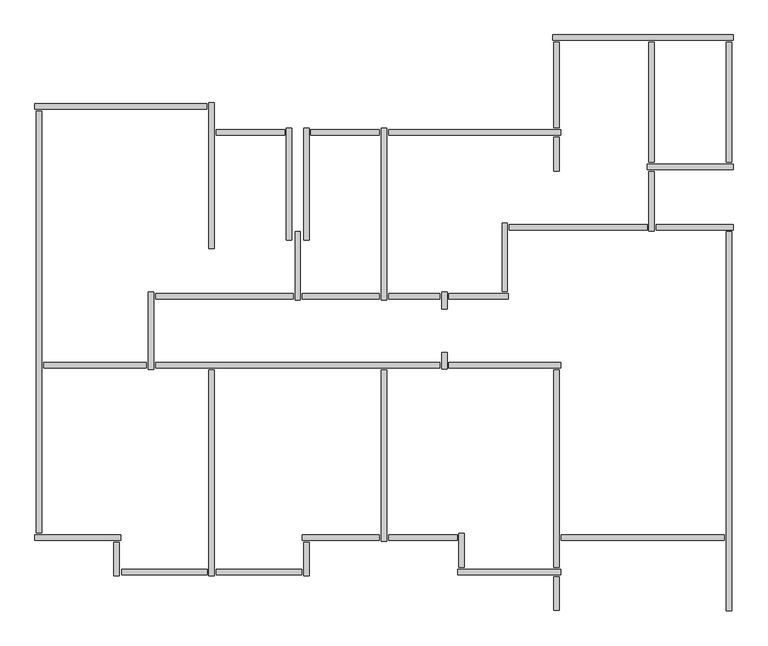
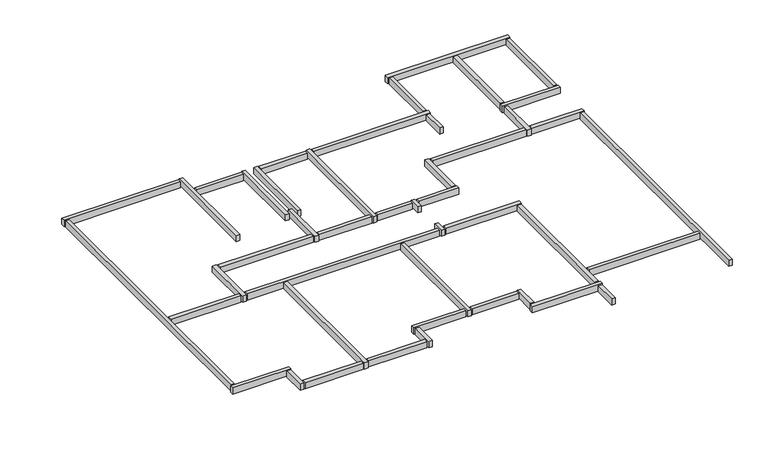
"""IFC4 building model written with IfcOpenShell, lengths in millimetres: beam geometry, Graute viga de respaldo2 : Graute viga de respaldo."""

import ifcopenshell
import ifcopenshell.guid

model = None  # the IFC model being written
_history = None  # IfcOwnerHistory: only IFC2X3 demands one
_inside = {}  # id of a spatial element -> (the spatial element, [elements in it])
_under = {}  # id of a project, library or spatial element -> (it, [spatial elements below it])
_declared = {}  # id of a project -> (the project, [libraries it declares])
_typed = {}  # id of a type object -> (the type object, [elements of that type])
_made_of = {}  # id of a material, layer set ... -> (it, [elements and type objects made of it])


def new_model(schema):
    """Start an empty IFC model of exactly this schema.

    Asked for "IFC4X3", IfcOpenShell would pick the latest addendum, in which some entities
    have other attributes; the version numbers below select the first issue.
    IFC2X3 requires an IfcOwnerHistory on every rooted entity: one is made here for all.
    """
    global model, _history
    if schema == "IFC4X3":
        model = ifcopenshell.file(schema_version=(4, 3, 0, 0))
    else:
        model = ifcopenshell.file(schema=schema)
    _inside.clear()
    _under.clear()
    _declared.clear()
    _typed.clear()
    _made_of.clear()
    _history = None
    if model.schema == "IFC2X3":
        org = make("IfcOrganization", Name="unknown")
        user = make(
            "IfcPersonAndOrganization",
            ThePerson=make("IfcPerson", FamilyName="unknown"),
            TheOrganization=org,
        )
        app = make(
            "IfcApplication",
            ApplicationDeveloper=org,
            Version="unknown",
            ApplicationFullName="unknown",
            ApplicationIdentifier="unknown",
        )
        _history = make(
            "IfcOwnerHistory",
            OwningUser=user,
            OwningApplication=app,
            ChangeAction="ADDED",
            CreationDate=0,
        )
    return model


def make(cls, **values):
    """One entity of the class cls with the attributes given. An attribute that is None is left unset."""
    return model.create_entity(
        cls, **{name: value for name, value in values.items() if value is not None}
    )


def rooted(cls, **values):
    """An entity with a GlobalId (a new one), such as an element, a storey or a relation."""
    return make(cls, GlobalId=ifcopenshell.guid.new(), OwnerHistory=_history, **values)


def si_unit(unit_type, name, prefix=None):
    """IfcSIUnit, for example si_unit("LENGTHUNIT", "METRE", prefix="MILLI")."""
    return make("IfcSIUnit", UnitType=unit_type, Prefix=prefix, Name=name)


def assignment(units):
    """IfcUnitAssignment: the units of a project."""
    return None if units is None else make("IfcUnitAssignment", Units=units)


def point(xyz):
    """IfcCartesianPoint."""
    return None if xyz is None else make("IfcCartesianPoint", Coordinates=xyz)


def direction(xyz):
    """IfcDirection."""
    return None if xyz is None else make("IfcDirection", DirectionRatios=xyz)


def frame(location, z_axis=None, x_axis=None):
    """IfcAxis2Placement3D, a coordinate frame: its origin and axes. An axis left out is left unset."""
    return make(
        "IfcAxis2Placement3D",
        Location=point(location),
        Axis=direction(z_axis),
        RefDirection=direction(x_axis),
    )


def origin():
    """The frame at (0, 0, 0) with its axes left unset."""
    return frame((0.0, 0.0, 0.0))


def place(relative_to, where):
    """IfcLocalPlacement: puts the frame where relative to a parent placement (None: the world)."""
    return make(
        "IfcLocalPlacement", PlacementRelTo=relative_to, RelativePlacement=where
    )


def context(
    kind, dimensions, precision=None, world=None, true_north=None, identifier=None
):
    """IfcGeometricRepresentationContext, for example the 3D "Model" context."""
    return make(
        "IfcGeometricRepresentationContext",
        ContextIdentifier=identifier,
        ContextType=kind,
        CoordinateSpaceDimension=dimensions,
        Precision=precision,
        WorldCoordinateSystem=world,
        TrueNorth=true_north,
    )


def project(units=None, contexts=None):
    """IfcProject with its units and contexts."""
    return rooted(
        "IfcProject",
        Name="project",
        RepresentationContexts=contexts,
        UnitsInContext=assignment(units),
    )


def spatial(cls, under=None, at=None, **own):
    """A site, building, storey or space (cls), placed at a placement, below another one or the project."""
    s = rooted(cls, ObjectPlacement=at, **own)
    if under is not None:
        _under.setdefault(under.id(), (under, []))[1].append(s)
    return s


def polyline(points):
    """IfcPolyline through the points."""
    return make("IfcPolyline", Points=[point(p) for p in points])


def outline(outer, holes=None, kind="AREA"):
    """IfcArbitraryClosedProfileDef: a profile drawn as a closed curve; with holes, ...WithVoids."""
    if holes is None:
        return make("IfcArbitraryClosedProfileDef", ProfileType=kind, OuterCurve=outer)
    return make(
        "IfcArbitraryProfileDefWithVoids",
        ProfileType=kind,
        OuterCurve=outer,
        InnerCurves=holes,
    )


def extrude(swept, where, along, depth):
    """IfcExtrudedAreaSolid: the profile swept, set in the frame where, extruded along a direction by depth."""
    return make(
        "IfcExtrudedAreaSolid",
        SweptArea=swept,
        Position=where,
        ExtrudedDirection=direction(along),
        Depth=depth,
    )


def shape(context_of_items, identifier, shape_type, items):
    """IfcShapeRepresentation: the items that make up one representation, for example the "Body"."""
    return make(
        "IfcShapeRepresentation",
        ContextOfItems=context_of_items,
        RepresentationIdentifier=identifier,
        RepresentationType=shape_type,
        Items=items,
    )


def source(mapping_origin, context_of_items, identifier, shape_type, items):
    """IfcRepresentationMap: a shape defined once, which mapped items show again and again."""
    return make(
        "IfcRepresentationMap",
        MappingOrigin=mapping_origin,
        MappedRepresentation=shape(context_of_items, identifier, shape_type, items),
    )


def transform(
    local_origin,
    x_axis=None,
    y_axis=None,
    z_axis=None,
    scale=None,
    scale2=None,
    scale3=None,
    uniform=True,
):
    """IfcCartesianTransformationOperator3D, or its non-uniform kind. x_axis, y_axis, z_axis: its Axis1, 2, 3."""
    if uniform:
        return make(
            "IfcCartesianTransformationOperator3D",
            Axis1=direction(x_axis),
            Axis2=direction(y_axis),
            LocalOrigin=point(local_origin),
            Scale=scale,
            Axis3=direction(z_axis),
        )
    return make(
        "IfcCartesianTransformationOperator3DnonUniform",
        Axis1=direction(x_axis),
        Axis2=direction(y_axis),
        LocalOrigin=point(local_origin),
        Scale=scale,
        Axis3=direction(z_axis),
        Scale2=scale2,
        Scale3=scale3,
    )


def mapped(mapping_source, mapping_target):
    """IfcMappedItem: shows the shape of a source again, moved by a transform."""
    return make(
        "IfcMappedItem", MappingSource=mapping_source, MappingTarget=mapping_target
    )


def made_of(thing, what):
    """Note that an element or type object is made of a material, layer set ...; save() writes the relation."""
    if what is not None:
        _made_of.setdefault(what.id(), (what, []))[1].append(thing)
    return thing


def element(
    cls,
    number,
    at=None,
    inside=None,
    cuts=None,
    type_object=None,
    material=None,
    context=None,
    identifier="Body",
    shape_type=None,
    held_by="IfcProductDefinitionShape",
    body=None,
    shapes=None,
    **own,
):
    """One element of the class cls, such as IfcWall. Its Tag is "e" and its number.

    at: its placement. inside: the storey or other place that contains it. cuts: it is an
    opening in that element (IfcRelVoidsElement). A single representation is given by context,
    identifier, shape_type and body (its items); several are given by shapes. held_by: the class
    of the entity that holds the representations. save() writes the other relations.
    """
    e = rooted(cls, Tag="e%d" % number, ObjectPlacement=at, **own)
    if body is not None:
        shapes = [shape(context, identifier, shape_type, body)]
    if shapes is not None:
        e.Representation = make(held_by, Representations=shapes)
    if inside is not None:
        _inside.setdefault(inside.id(), (inside, []))[1].append(e)
    if cuts is not None:
        rooted(
            "IfcRelVoidsElement", RelatingBuildingElement=cuts, RelatedOpeningElement=e
        )
    if type_object is not None:
        _typed.setdefault(type_object.id(), (type_object, []))[1].append(e)
    return made_of(e, material)


def aggregate(whole, parts):
    """IfcRelAggregates: a whole, such as a stair, and the parts it consists of."""
    return rooted("IfcRelAggregates", RelatingObject=whole, RelatedObjects=parts)


def save(model, path):
    """Write the relations noted so far, then the file.

    IfcRelAggregates (storeys below a building ...), IfcRelContainedInSpatialStructure (elements
    in a storey), IfcRelDefinesByType, IfcRelAssociatesMaterial and IfcRelDeclares: one each for
    every whole, place, type object, material and project.
    """
    for whole, parts in _under.values():
        aggregate(whole, parts)
    for where, things in _inside.values():
        rooted(
            "IfcRelContainedInSpatialStructure",
            RelatedElements=things,
            RelatingStructure=where,
        )
    for kind, things in _typed.values():
        rooted("IfcRelDefinesByType", RelatedObjects=things, RelatingType=kind)
    for what, things in _made_of.values():
        rooted("IfcRelAssociatesMaterial", RelatedObjects=things, RelatingMaterial=what)
    for by, libraries in _declared.values():
        rooted("IfcRelDeclares", RelatingContext=by, RelatedDefinitions=libraries)
    model.write(path)


def beam_834ff979(model_context):
    return source(origin(), model_context, "Body", "SweptSolid", [
        extrude(outline(polyline([(-75401.7587292, 57502.4278788), (-75401.7587292, 57408.4278788), (-76591.7587292, 57408.4278788), (-76591.7587292, 57502.4278788), (-75401.7587292, 57502.4278788)])), frame((0.0, 0.0, 2632.9999999), z_axis=(0.0, 0.0, 1.0), x_axis=(1.0, 0.0, 0.0)), (0.0, 0.0, 1.0), 167.0),
        extrude(outline(polyline([(-73751.7587292, 57502.4278788), (-73751.7587292, 57408.4278788), (-74941.7587292, 57408.4278788), (-74941.7587292, 57502.4278788), (-73751.7587292, 57502.4278788)])), frame((0.0, 0.0, 2632.9999999), z_axis=(0.0, 0.0, 1.0), x_axis=(1.0, 0.0, 0.0)), (0.0, 0.0, 1.0), 167.0),
        extrude(outline(polyline([(-77801.7587292, 53452.4278788), (-77801.7587292, 53358.4278788), (-79591.7587292, 53358.4278788), (-79591.7587292, 53452.4278788), (-77801.7587292, 53452.4278788)])), frame((0.0, 0.0, 2632.9999999), z_axis=(0.0, 0.0, 1.0), x_axis=(1.0, 0.0, 0.0)), (0.0, 0.0, 1.0), 167.0),
        extrude(outline(polyline([(-72401.7587292, 50452.4278788), (-72401.7587292, 50358.4278788), (-73591.7587292, 50358.4278788), (-73591.7587292, 50452.4278788), (-72401.7587292, 50452.4278788)])), frame((0.0, 0.0, 2632.9999999), z_axis=(0.0, 0.0, 1.0), x_axis=(1.0, 0.0, 0.0)), (0.0, 0.0, 1.0), 167.0),
        extrude(outline(polyline([(-72368.7587292, 50475.4278788), (-72274.7587292, 50475.4278788), (-72274.7587292, 49885.4278788), (-72368.7587292, 49885.4278788), (-72368.7587292, 50475.4278788)])), frame((0.0, 0.0, 2632.9999999), z_axis=(0.0, 0.0, 1.0), x_axis=(1.0, 0.0, 0.0)), (0.0, 0.0, 1.0), 167.0),
        extrude(outline(polyline([(-70601.7587292, 49852.4278788), (-70601.7587292, 49758.4278788), (-72391.7587292, 49758.4278788), (-72391.7587292, 49852.4278788), (-70601.7587292, 49852.4278788)])), frame((0.0, 0.0, 2632.9999999), z_axis=(0.0, 0.0, 1.0), x_axis=(1.0, 0.0, 0.0)), (0.0, 0.0, 1.0), 167.0),
        extrude(outline(polyline([(-72574.7587292, 53335.4278788), (-72668.7587292, 53335.4278788), (-72668.7587292, 53625.4278788), (-72574.7587292, 53625.4278788), (-72574.7587292, 53335.4278788)])), frame((0.0, 0.0, 2632.9999999), z_axis=(0.0, 0.0, 1.0), x_axis=(1.0, 0.0, 0.0)), (0.0, 0.0, 1.0), 167.0),
        extrude(outline(polyline([(-75251.7587292, 54652.4278788), (-75251.7587292, 54558.4278788), (-77641.7587292, 54558.4278788), (-77641.7587292, 54652.4278788), (-75251.7587292, 54652.4278788)])), frame((0.0, 0.0, 2632.9999999), z_axis=(0.0, 0.0, 1.0), x_axis=(1.0, 0.0, 0.0)), (0.0, 0.0, 1.0), 167.0),
        extrude(outline(polyline([(-73751.7587292, 54652.4278788), (-73751.7587292, 54558.4278788), (-75091.7587292, 54558.4278788), (-75091.7587292, 54652.4278788), (-73751.7587292, 54652.4278788)])), frame((0.0, 0.0, 2632.9999999), z_axis=(0.0, 0.0, 1.0), x_axis=(1.0, 0.0, 0.0)), (0.0, 0.0, 1.0), 167.0),
        extrude(outline(polyline([(-72701.7587292, 54652.4278788), (-72701.7587292, 54558.4278788), (-73591.7587292, 54558.4278788), (-73591.7587292, 54652.4278788), (-72701.7587292, 54652.4278788)])), frame((0.0, 0.0, 2632.9999999), z_axis=(0.0, 0.0, 1.0), x_axis=(1.0, 0.0, 0.0)), (0.0, 0.0, 1.0), 167.0),
        extrude(outline(polyline([(-72574.7587292, 54385.4278788), (-72668.7587292, 54385.4278788), (-72668.7587292, 54675.4278788), (-72574.7587292, 54675.4278788), (-72574.7587292, 54385.4278788)])), frame((0.0, 0.0, 2632.9999999), z_axis=(0.0, 0.0, 1.0), x_axis=(1.0, 0.0, 0.0)), (0.0, 0.0, 1.0), 167.0),
        extrude(outline(polyline([(-71511.7587292, 54652.4278788), (-71511.7587292, 54558.4278788), (-72541.7587292, 54558.4278788), (-72541.7587292, 54652.4278788), (-71511.7587292, 54652.4278788)])), frame((0.0, 0.0, 2632.9999999), z_axis=(0.0, 0.0, 1.0), x_axis=(1.0, 0.0, 0.0)), (0.0, 0.0, 1.0), 167.0),
        extrude(outline(polyline([(-71618.7587292, 55875.4278788), (-71524.7587292, 55875.4278788), (-71524.7587292, 54685.4278788), (-71618.7587292, 54685.4278788), (-71618.7587292, 55875.4278788)])), frame((0.0, 0.0, 2632.9999999), z_axis=(0.0, 0.0, 1.0), x_axis=(1.0, 0.0, 0.0)), (0.0, 0.0, 1.0), 167.0),
        extrude(outline(polyline([(-69091.7587292, 55852.4278788), (-69091.7587292, 55758.4278788), (-71491.7587292, 55758.4278788), (-71491.7587292, 55852.4278788), (-69091.7587292, 55852.4278788)])), frame((0.0, 0.0, 2632.9999999), z_axis=(0.0, 0.0, 1.0), x_axis=(1.0, 0.0, 0.0)), (0.0, 0.0, 1.0), 167.0),
        extrude(outline(polyline([(-73624.7587292, 54540.4278788), (-73718.7587292, 54540.4278788), (-73718.7587292, 57525.4278788), (-73624.7587292, 57525.4278788), (-73624.7587292, 54540.4278788)])), frame((0.0, 0.0, 2632.9999999), z_axis=(0.0, 0.0, 1.0), x_axis=(1.0, 0.0, 0.0)), (0.0, 0.0, 1.0), 167.0),
        extrude(outline(polyline([(-70601.7587292, 57502.4278788), (-70601.7587292, 57408.4278788), (-73591.7587292, 57408.4278788), (-73591.7587292, 57502.4278788), (-70601.7587292, 57502.4278788)])), frame((0.0, 0.0, 2632.9999999), z_axis=(0.0, 0.0, 1.0), x_axis=(1.0, 0.0, 0.0)), (0.0, 0.0, 1.0), 167.0),
        extrude(outline(polyline([(-70624.7587292, 56785.4278788), (-70718.7587292, 56785.4278788), (-70718.7587292, 57375.4278788), (-70624.7587292, 57375.4278788), (-70624.7587292, 56785.4278788)])), frame((0.0, 0.0, 2632.9999999), z_axis=(0.0, 0.0, 1.0), x_axis=(1.0, 0.0, 0.0)), (0.0, 0.0, 1.0), 167.0),
        extrude(outline(polyline([(-70718.7587292, 59025.4278788), (-70624.7587292, 59025.4278788), (-70624.7587292, 57535.4278788), (-70718.7587292, 57535.4278788), (-70718.7587292, 59025.4278788)])), frame((0.0, 0.0, 2632.9999999), z_axis=(0.0, 0.0, 1.0), x_axis=(1.0, 0.0, 0.0)), (0.0, 0.0, 1.0), 167.0),
        extrude(outline(polyline([(-67718.7587292, 59025.4278788), (-67624.7587292, 59025.4278788), (-67624.7587292, 56935.4278788), (-67718.7587292, 56935.4278788), (-67718.7587292, 59025.4278788)])), frame((0.0, 0.0, 2632.9999999), z_axis=(0.0, 0.0, 1.0), x_axis=(1.0, 0.0, 0.0)), (0.0, 0.0, 1.0), 167.0),
        extrude(outline(polyline([(-69068.7587292, 59025.4278788), (-68974.7587292, 59025.4278788), (-68974.7587292, 56935.4278788), (-69068.7587292, 56935.4278788), (-69068.7587292, 59025.4278788)])), frame((0.0, 0.0, 2632.9999999), z_axis=(0.0, 0.0, 1.0), x_axis=(1.0, 0.0, 0.0)), (0.0, 0.0, 1.0), 167.0),
        extrude(outline(polyline([(-68974.7587292, 55735.4278788), (-69068.7587292, 55735.4278788), (-69068.7587292, 56775.4278788), (-68974.7587292, 56775.4278788), (-68974.7587292, 55735.4278788)])), frame((0.0, 0.0, 2632.9999999), z_axis=(0.0, 0.0, 1.0), x_axis=(1.0, 0.0, 0.0)), (0.0, 0.0, 1.0), 167.0),
        extrude(outline(polyline([(-67751.7587292, 50452.4278788), (-67751.7587292, 50358.4278788), (-70591.7587292, 50358.4278788), (-70591.7587292, 50452.4278788), (-67751.7587292, 50452.4278788)])), frame((0.0, 0.0, 2632.9999999), z_axis=(0.0, 0.0, 1.0), x_axis=(1.0, 0.0, 0.0)), (0.0, 0.0, 1.0), 167.0),
        extrude(outline(polyline([(-70718.7587292, 53325.4278788), (-70624.7587292, 53325.4278788), (-70624.7587292, 49885.4278788), (-70718.7587292, 49885.4278788), (-70718.7587292, 53325.4278788)])), frame((0.0, 0.0, 2632.9999999), z_axis=(0.0, 0.0, 1.0), x_axis=(1.0, 0.0, 0.0)), (0.0, 0.0, 1.0), 167.0),
        extrude(outline(polyline([(-70601.7587292, 53452.4278788), (-70601.7587292, 53358.4278788), (-72541.7587292, 53358.4278788), (-72541.7587292, 53452.4278788), (-70601.7587292, 53452.4278788)])), frame((0.0, 0.0, 2632.9999999), z_axis=(0.0, 0.0, 1.0), x_axis=(1.0, 0.0, 0.0)), (0.0, 0.0, 1.0), 167.0),
        extrude(outline(polyline([(-72701.7587292, 53452.4278788), (-72701.7587292, 53358.4278788), (-77641.7587292, 53358.4278788), (-77641.7587292, 53452.4278788), (-72701.7587292, 53452.4278788)])), frame((0.0, 0.0, 2632.9999999), z_axis=(0.0, 0.0, 1.0), x_axis=(1.0, 0.0, 0.0)), (0.0, 0.0, 1.0), 167.0),
        extrude(outline(polyline([(-73624.7587292, 50335.4278788), (-73718.7587292, 50335.4278788), (-73718.7587292, 53325.4278788), (-73624.7587292, 53325.4278788), (-73624.7587292, 50335.4278788)])), frame((0.0, 0.0, 2632.9999999), z_axis=(0.0, 0.0, 1.0), x_axis=(1.0, 0.0, 0.0)), (0.0, 0.0, 1.0), 167.0),
        extrude(outline(polyline([(-75091.7587292, 50358.4278788), (-75091.7587292, 50452.4278788), (-73751.7587292, 50452.4278788), (-73751.7587292, 50358.4278788), (-75091.7587292, 50358.4278788)])), frame((0.0, 0.0, 2632.9999999), z_axis=(0.0, 0.0, 1.0), x_axis=(1.0, 0.0, 0.0)), (0.0, 0.0, 1.0), 167.0),
        extrude(outline(polyline([(-74974.7587292, 49735.4278788), (-75068.7587292, 49735.4278788), (-75068.7587292, 50325.4278788), (-74974.7587292, 50325.4278788), (-74974.7587292, 49735.4278788)])), frame((0.0, 0.0, 2632.9999999), z_axis=(0.0, 0.0, 1.0), x_axis=(1.0, 0.0, 0.0)), (0.0, 0.0, 1.0), 167.0),
        extrude(outline(polyline([(-75101.7587292, 49852.4278788), (-75101.7587292, 49758.4278788), (-76591.7587292, 49758.4278788), (-76591.7587292, 49852.4278788), (-75101.7587292, 49852.4278788)])), frame((0.0, 0.0, 2632.9999999), z_axis=(0.0, 0.0, 1.0), x_axis=(1.0, 0.0, 0.0)), (0.0, 0.0, 1.0), 167.0),
        extrude(outline(polyline([(-78230.736554, 49758.4278788), (-78230.736554, 49853.4278788), (-76741.7587292, 49853.4278788), (-76741.7587292, 49758.4278788), (-78230.736554, 49758.4278788)])), frame((0.0, 0.0, 2617.1856208), z_axis=(0.0, 0.0, 1.0), x_axis=(1.0, 0.0, 0.0)), (0.0, 0.0, 1.0), 165.0),
        extrude(outline(polyline([(-79718.7587292, 57825.4278788), (-79624.7587292, 57825.4278788), (-79624.7587292, 50485.4278788), (-79718.7587292, 50485.4278788), (-79718.7587292, 57825.4278788)])), frame((0.0, 0.0, 2632.9999999), z_axis=(0.0, 0.0, 1.0), x_axis=(1.0, 0.0, 0.0)), (0.0, 0.0, 1.0), 167.0),
        extrude(outline(polyline([(-77768.7587292, 54675.4278788), (-77674.7587292, 54675.4278788), (-77674.7587292, 53330.0746661), (-77768.7587292, 53330.0746661), (-77768.7587292, 54675.4278788)])), frame((0.0, 0.0, 2632.9999999), z_axis=(0.0, 0.0, 1.0), x_axis=(1.0, 0.0, 0.0)), (0.0, 0.0, 1.0), 167.0),
        extrude(outline(polyline([(-75218.7587292, 55725.4278788), (-75124.7587292, 55725.4278788), (-75124.7587292, 54535.4278788), (-75218.7587292, 54535.4278788), (-75218.7587292, 55725.4278788)])), frame((0.0, 0.0, 2632.9999999), z_axis=(0.0, 0.0, 1.0), x_axis=(1.0, 0.0, 0.0)), (0.0, 0.0, 1.0), 167.0),
        extrude(outline(polyline([(-75368.7587292, 57525.4278788), (-75274.7587292, 57525.4278788), (-75274.7587292, 55585.4278788), (-75368.7587292, 55585.4278788), (-75368.7587292, 57525.4278788)])), frame((0.0, 0.0, 2632.9999999), z_axis=(0.0, 0.0, 1.0), x_axis=(1.0, 0.0, 0.0)), (0.0, 0.0, 1.0), 167.0),
        extrude(outline(polyline([(-75068.7587292, 57525.4278788), (-74974.7587292, 57525.4278788), (-74974.7587292, 55585.4278788), (-75068.7587292, 55585.4278788), (-75068.7587292, 57525.4278788)])), frame((0.0, 0.0, 2632.9999999), z_axis=(0.0, 0.0, 1.0), x_axis=(1.0, 0.0, 0.0)), (0.0, 0.0, 1.0), 167.0),
        extrude(outline(polyline([(-76718.7587292, 57975.4278788), (-76624.7587292, 57975.4278788), (-76624.7587292, 55435.4278788), (-76718.7587292, 55435.4278788), (-76718.7587292, 57975.4278788)])), frame((0.0, 0.0, 2632.9999999), z_axis=(0.0, 0.0, 1.0), x_axis=(1.0, 0.0, 0.0)), (0.0, 0.0, 1.0), 167.0),
        extrude(outline(polyline([(-79741.7587292, 57858.4278788), (-79741.7587292, 57952.4278788), (-76751.7587292, 57952.4278788), (-76751.7587292, 57858.4278788), (-79741.7587292, 57858.4278788)])), frame((0.0, 0.0, 2632.9999999), z_axis=(0.0, 0.0, 1.0), x_axis=(1.0, 0.0, 0.0)), (0.0, 0.0, 1.0), 167.0),
        extrude(outline(polyline([(-78274.7587292, 49735.4278788), (-78368.7587292, 49735.4278788), (-78368.7587292, 50325.4278788), (-78274.7587292, 50325.4278788), (-78274.7587292, 49735.4278788)])), frame((0.0, 0.0, 2632.9999999), z_axis=(0.0, 0.0, 1.0), x_axis=(1.0, 0.0, 0.0)), (0.0, 0.0, 1.0), 167.0),
        extrude(outline(polyline([(-78251.7587292, 50452.4278788), (-78251.7587292, 50358.4278788), (-79741.7587292, 50358.4278788), (-79741.7587292, 50452.4278788), (-78251.7587292, 50452.4278788)])), frame((0.0, 0.0, 2632.9999999), z_axis=(0.0, 0.0, 1.0), x_axis=(1.0, 0.0, 0.0)), (0.0, 0.0, 1.0), 167.0),
        extrude(outline(polyline([(-76624.7587292, 49735.4278788), (-76718.7587292, 49735.4278788), (-76718.7587292, 53325.4278788), (-76624.7587292, 53325.4278788), (-76624.7587292, 49735.4278788)])), frame((0.0, 0.0, 2632.9999999), z_axis=(0.0, 0.0, 1.0), x_axis=(1.0, 0.0, 0.0)), (0.0, 0.0, 1.0), 167.0),
        extrude(outline(polyline([(-70624.7587292, 49135.4278788), (-70718.7587292, 49135.4278788), (-70718.7587292, 49725.4278788), (-70624.7587292, 49725.4278788), (-70624.7587292, 49135.4278788)])), frame((0.0, 0.0, 2632.9999999), z_axis=(0.0, 0.0, 1.0), x_axis=(1.0, 0.0, 0.0)), (0.0, 0.0, 1.0), 167.0),
        extrude(outline(polyline([(-67601.7587292, 56902.4278788), (-67601.7587292, 56808.4278788), (-69091.7587292, 56808.4278788), (-69091.7587292, 56902.4278788), (-67601.7587292, 56902.4278788)])), frame((0.0, 0.0, 2632.9999999), z_axis=(0.0, 0.0, 1.0), x_axis=(1.0, 0.0, 0.0)), (0.0, 0.0, 1.0), 167.0),
        extrude(outline(polyline([(-67601.7587292, 59152.4278788), (-67601.7587292, 59058.4278788), (-70741.7587292, 59058.4278788), (-70741.7587292, 59152.4278788), (-67601.7587292, 59152.4278788)])), frame((0.0, 0.0, 2632.9999999), z_axis=(0.0, 0.0, 1.0), x_axis=(1.0, 0.0, 0.0)), (0.0, 0.0, 1.0), 167.0),
        extrude(outline(polyline([(-67601.7587292, 55852.4278788), (-67601.7587292, 55758.4278788), (-68941.7587292, 55758.4278788), (-68941.7587292, 55852.4278788), (-67601.7587292, 55852.4278788)])), frame((0.0, 0.0, 2632.9999999), z_axis=(0.0, 0.0, 1.0), x_axis=(1.0, 0.0, 0.0)), (0.0, 0.0, 1.0), 167.0),
        extrude(outline(polyline([(-67624.7587292, 49132.8979841), (-67718.7587292, 49132.8979841), (-67718.7587292, 55725.4278788), (-67624.7587292, 55725.4278788), (-67624.7587292, 49132.8979841)])), frame((0.0, 0.0, 2632.9999999), z_axis=(0.0, 0.0, 1.0), x_axis=(1.0, 0.0, 0.0)), (0.0, 0.0, 1.0), 167.0),
    ])


if __name__ == "__main__":
    model = new_model("IFC4")
    model_context = context("Model", 3, world=origin())
    ifc_project = project(units=[si_unit("LENGTHUNIT", "METRE", prefix="MILLI")], contexts=[model_context])
    site = spatial("IfcSite", under=ifc_project)
    building = spatial("IfcBuilding", under=site)
    placement = place(None, origin())
    beam_shape = beam_834ff979(model_context)
    element("IfcBeam", 1, ObjectType="Graute viga de respaldo2 : Graute viga de respaldo", at=placement, inside=building, context=model_context, shape_type="MappedRepresentation", body=[
        mapped(beam_shape, transform((0.0, 0.0, 0.0), x_axis=(1.0, 0.0, 0.0), y_axis=(0.0, 1.0, 0.0), z_axis=(0.0, 0.0, 1.0))),
    ])
    save(model, "model.ifc")

# Revit data of these elements
# Element 1 (IfcBeam, "Graute viga de respaldo2 : Graute viga de respaldo")
#   Materials on its faces: "Concreto, Faixa de areia/cimento"
# Materials
#   "Concreto, Faixa de areia/cimento": class "Concreto", colour RGB 127 127 127, transparency 0, Description = "Revestimento de laje de concreto", Cost = 0
